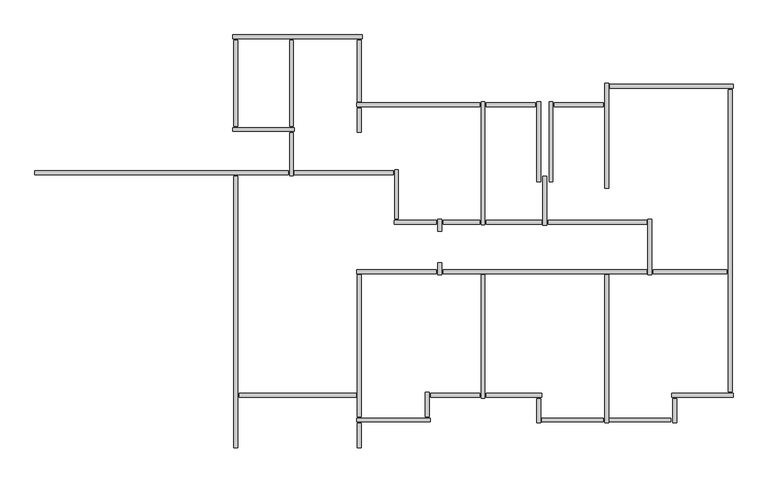
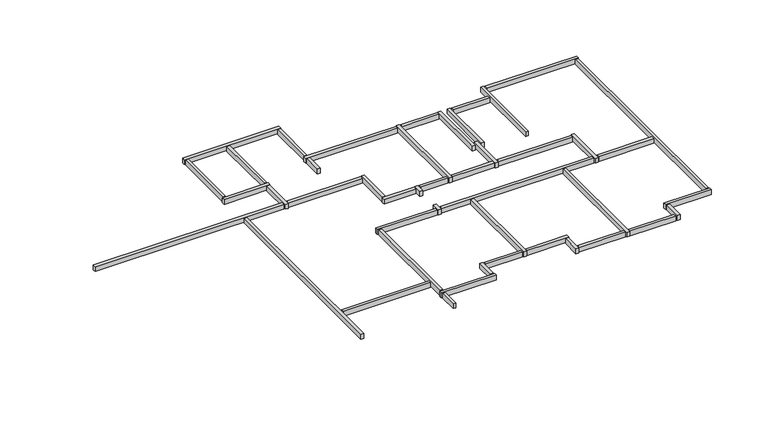
"""IFC4 building model written with IfcOpenShell, lengths in millimetres: beam geometry, Graute viga de respaldo4 : Graute viga de respaldo."""

from ifc_helpers import new_model, si_unit, frame, origin, place, context, project, spatial, polyline, outline, extrude, source, transform, mapped, element, save


def beam_ccfebb10(model_context):
    return source(origin(), model_context, "Body", "SweptSolid", [
        extrude(outline(polyline([(-54994.9587292, 57408.4278788), (-54994.9587292, 57502.4278788), (-53804.9587292, 57502.4278788), (-53804.9587292, 57408.4278788), (-54994.9587292, 57408.4278788)])), frame((0.0, 0.0, 5632.9999999), z_axis=(0.0, 0.0, 1.0), x_axis=(1.0, 0.0, 0.0)), (0.0, 0.0, 1.0), 167.0),
        extrude(outline(polyline([(-56644.9587292, 57408.4278788), (-56644.9587292, 57502.4278788), (-55454.9587292, 57502.4278788), (-55454.9587292, 57408.4278788), (-56644.9587292, 57408.4278788)])), frame((0.0, 0.0, 5632.9999999), z_axis=(0.0, 0.0, 1.0), x_axis=(1.0, 0.0, 0.0)), (0.0, 0.0, 1.0), 167.0),
        extrude(outline(polyline([(-52594.9587292, 53358.4278788), (-52594.9587292, 53452.4278788), (-50804.9587292, 53452.4278788), (-50804.9587292, 53358.4278788), (-52594.9587292, 53358.4278788)])), frame((0.0, 0.0, 5632.9999999), z_axis=(0.0, 0.0, 1.0), x_axis=(1.0, 0.0, 0.0)), (0.0, 0.0, 1.0), 167.0),
        extrude(outline(polyline([(-57994.9587292, 50358.4278788), (-57994.9587292, 50452.4278788), (-56804.9587292, 50452.4278788), (-56804.9587292, 50358.4278788), (-57994.9587292, 50358.4278788)])), frame((0.0, 0.0, 5632.9999999), z_axis=(0.0, 0.0, 1.0), x_axis=(1.0, 0.0, 0.0)), (0.0, 0.0, 1.0), 167.0),
        extrude(outline(polyline([(-58121.9587292, 50475.4278788), (-58027.9587292, 50475.4278788), (-58027.9587292, 49885.4278788), (-58121.9587292, 49885.4278788), (-58121.9587292, 50475.4278788)])), frame((0.0, 0.0, 5632.9999999), z_axis=(0.0, 0.0, 1.0), x_axis=(1.0, 0.0, 0.0)), (0.0, 0.0, 1.0), 167.0),
        extrude(outline(polyline([(-59794.9587292, 49758.4278788), (-59794.9587292, 49852.4278788), (-58004.9587292, 49852.4278788), (-58004.9587292, 49758.4278788), (-59794.9587292, 49758.4278788)])), frame((0.0, 0.0, 5632.9999999), z_axis=(0.0, 0.0, 1.0), x_axis=(1.0, 0.0, 0.0)), (0.0, 0.0, 1.0), 167.0),
        extrude(outline(polyline([(-57727.9587292, 53335.4278788), (-57821.9587292, 53335.4278788), (-57821.9587292, 53625.4278788), (-57727.9587292, 53625.4278788), (-57727.9587292, 53335.4278788)])), frame((0.0, 0.0, 5632.9999999), z_axis=(0.0, 0.0, 1.0), x_axis=(1.0, 0.0, 0.0)), (0.0, 0.0, 1.0), 167.0),
        extrude(outline(polyline([(-55144.9587292, 54558.4278788), (-55144.9587292, 54652.4278788), (-52754.9587292, 54652.4278788), (-52754.9587292, 54558.4278788), (-55144.9587292, 54558.4278788)])), frame((0.0, 0.0, 5632.9999999), z_axis=(0.0, 0.0, 1.0), x_axis=(1.0, 0.0, 0.0)), (0.0, 0.0, 1.0), 167.0),
        extrude(outline(polyline([(-56644.9587292, 54558.4278788), (-56644.9587292, 54652.4278788), (-55304.9587292, 54652.4278788), (-55304.9587292, 54558.4278788), (-56644.9587292, 54558.4278788)])), frame((0.0, 0.0, 5632.9999999), z_axis=(0.0, 0.0, 1.0), x_axis=(1.0, 0.0, 0.0)), (0.0, 0.0, 1.0), 167.0),
        extrude(outline(polyline([(-57694.9587292, 54558.4278788), (-57694.9587292, 54652.4278788), (-56804.9587292, 54652.4278788), (-56804.9587292, 54558.4278788), (-57694.9587292, 54558.4278788)])), frame((0.0, 0.0, 5632.9999999), z_axis=(0.0, 0.0, 1.0), x_axis=(1.0, 0.0, 0.0)), (0.0, 0.0, 1.0), 167.0),
        extrude(outline(polyline([(-57727.9587292, 54385.4278788), (-57821.9587292, 54385.4278788), (-57821.9587292, 54675.4278788), (-57727.9587292, 54675.4278788), (-57727.9587292, 54385.4278788)])), frame((0.0, 0.0, 5632.9999999), z_axis=(0.0, 0.0, 1.0), x_axis=(1.0, 0.0, 0.0)), (0.0, 0.0, 1.0), 167.0),
        extrude(outline(polyline([(-58884.9587292, 54558.4278788), (-58884.9587292, 54652.4278788), (-57854.9587292, 54652.4278788), (-57854.9587292, 54558.4278788), (-58884.9587292, 54558.4278788)])), frame((0.0, 0.0, 5632.9999999), z_axis=(0.0, 0.0, 1.0), x_axis=(1.0, 0.0, 0.0)), (0.0, 0.0, 1.0), 167.0),
        extrude(outline(polyline([(-58871.9587292, 55875.4278788), (-58777.9587292, 55875.4278788), (-58777.9587292, 54685.4278788), (-58871.9587292, 54685.4278788), (-58871.9587292, 55875.4278788)])), frame((0.0, 0.0, 5632.9999999), z_axis=(0.0, 0.0, 1.0), x_axis=(1.0, 0.0, 0.0)), (0.0, 0.0, 1.0), 167.0),
        extrude(outline(polyline([(-61304.9587292, 55758.4278788), (-61304.9587292, 55852.4278788), (-58904.9587292, 55852.4278788), (-58904.9587292, 55758.4278788), (-61304.9587292, 55758.4278788)])), frame((0.0, 0.0, 5632.9999999), z_axis=(0.0, 0.0, 1.0), x_axis=(1.0, 0.0, 0.0)), (0.0, 0.0, 1.0), 167.0),
        extrude(outline(polyline([(-56677.9587292, 54540.4278788), (-56771.9587292, 54540.4278788), (-56771.9587292, 57525.4278788), (-56677.9587292, 57525.4278788), (-56677.9587292, 54540.4278788)])), frame((0.0, 0.0, 5632.9999999), z_axis=(0.0, 0.0, 1.0), x_axis=(1.0, 0.0, 0.0)), (0.0, 0.0, 1.0), 167.0),
        extrude(outline(polyline([(-59794.9587292, 57408.4278788), (-59794.9587292, 57502.4278788), (-56804.9587292, 57502.4278788), (-56804.9587292, 57408.4278788), (-59794.9587292, 57408.4278788)])), frame((0.0, 0.0, 5632.9999999), z_axis=(0.0, 0.0, 1.0), x_axis=(1.0, 0.0, 0.0)), (0.0, 0.0, 1.0), 167.0),
        extrude(outline(polyline([(-59677.9587292, 56785.4278788), (-59771.9587292, 56785.4278788), (-59771.9587292, 57375.4278788), (-59677.9587292, 57375.4278788), (-59677.9587292, 56785.4278788)])), frame((0.0, 0.0, 5632.9999999), z_axis=(0.0, 0.0, 1.0), x_axis=(1.0, 0.0, 0.0)), (0.0, 0.0, 1.0), 167.0),
        extrude(outline(polyline([(-59771.9587292, 59025.4278788), (-59677.9587292, 59025.4278788), (-59677.9587292, 57535.4278788), (-59771.9587292, 57535.4278788), (-59771.9587292, 59025.4278788)])), frame((0.0, 0.0, 5632.9999999), z_axis=(0.0, 0.0, 1.0), x_axis=(1.0, 0.0, 0.0)), (0.0, 0.0, 1.0), 167.0),
        extrude(outline(polyline([(-62771.9587292, 59025.4278788), (-62677.9587292, 59025.4278788), (-62677.9587292, 56935.4278788), (-62771.9587292, 56935.4278788), (-62771.9587292, 59025.4278788)])), frame((0.0, 0.0, 5632.9999999), z_axis=(0.0, 0.0, 1.0), x_axis=(1.0, 0.0, 0.0)), (0.0, 0.0, 1.0), 167.0),
        extrude(outline(polyline([(-61421.9587292, 59025.4278788), (-61327.9587292, 59025.4278788), (-61327.9587292, 56935.4278788), (-61421.9587292, 56935.4278788), (-61421.9587292, 59025.4278788)])), frame((0.0, 0.0, 5632.9999999), z_axis=(0.0, 0.0, 1.0), x_axis=(1.0, 0.0, 0.0)), (0.0, 0.0, 1.0), 167.0),
        extrude(outline(polyline([(-61327.9587292, 55735.4278788), (-61421.9587292, 55735.4278788), (-61421.9587292, 56775.4278788), (-61327.9587292, 56775.4278788), (-61327.9587292, 55735.4278788)])), frame((0.0, 0.0, 5632.9999999), z_axis=(0.0, 0.0, 1.0), x_axis=(1.0, 0.0, 0.0)), (0.0, 0.0, 1.0), 167.0),
        extrude(outline(polyline([(-62644.9587292, 50358.4278788), (-62644.9587292, 50452.4278788), (-59804.9587292, 50452.4278788), (-59804.9587292, 50358.4278788), (-62644.9587292, 50358.4278788)])), frame((0.0, 0.0, 5632.9999999), z_axis=(0.0, 0.0, 1.0), x_axis=(1.0, 0.0, 0.0)), (0.0, 0.0, 1.0), 167.0),
        extrude(outline(polyline([(-59771.9587292, 53325.4278788), (-59677.9587292, 53325.4278788), (-59677.9587292, 49885.4278788), (-59771.9587292, 49885.4278788), (-59771.9587292, 53325.4278788)])), frame((0.0, 0.0, 5632.9999999), z_axis=(0.0, 0.0, 1.0), x_axis=(1.0, 0.0, 0.0)), (0.0, 0.0, 1.0), 167.0),
        extrude(outline(polyline([(-59794.9587292, 53358.4278788), (-59794.9587292, 53452.4278788), (-57854.9587292, 53452.4278788), (-57854.9587292, 53358.4278788), (-59794.9587292, 53358.4278788)])), frame((0.0, 0.0, 5632.9999999), z_axis=(0.0, 0.0, 1.0), x_axis=(1.0, 0.0, 0.0)), (0.0, 0.0, 1.0), 167.0),
        extrude(outline(polyline([(-57694.9587292, 53358.4278788), (-57694.9587292, 53452.4278788), (-52754.9587292, 53452.4278788), (-52754.9587292, 53358.4278788), (-57694.9587292, 53358.4278788)])), frame((0.0, 0.0, 5632.9999999), z_axis=(0.0, 0.0, 1.0), x_axis=(1.0, 0.0, 0.0)), (0.0, 0.0, 1.0), 167.0),
        extrude(outline(polyline([(-56677.9587292, 50335.4278788), (-56771.9587292, 50335.4278788), (-56771.9587292, 53325.4278788), (-56677.9587292, 53325.4278788), (-56677.9587292, 50335.4278788)])), frame((0.0, 0.0, 5632.9999999), z_axis=(0.0, 0.0, 1.0), x_axis=(1.0, 0.0, 0.0)), (0.0, 0.0, 1.0), 167.0),
        extrude(outline(polyline([(-55304.9587292, 50452.4278788), (-55304.9587292, 50358.4278788), (-56644.9587292, 50358.4278788), (-56644.9587292, 50452.4278788), (-55304.9587292, 50452.4278788)])), frame((0.0, 0.0, 5632.9999999), z_axis=(0.0, 0.0, 1.0), x_axis=(1.0, 0.0, 0.0)), (0.0, 0.0, 1.0), 167.0),
        extrude(outline(polyline([(-55327.9587292, 49735.4278788), (-55421.9587292, 49735.4278788), (-55421.9587292, 50325.4278788), (-55327.9587292, 50325.4278788), (-55327.9587292, 49735.4278788)])), frame((0.0, 0.0, 5632.9999999), z_axis=(0.0, 0.0, 1.0), x_axis=(1.0, 0.0, 0.0)), (0.0, 0.0, 1.0), 167.0),
        extrude(outline(polyline([(-55294.9587292, 49758.4278788), (-55294.9587292, 49852.4278788), (-53804.9587292, 49852.4278788), (-53804.9587292, 49758.4278788), (-55294.9587292, 49758.4278788)])), frame((0.0, 0.0, 5632.9999999), z_axis=(0.0, 0.0, 1.0), x_axis=(1.0, 0.0, 0.0)), (0.0, 0.0, 1.0), 167.0),
        extrude(outline(polyline([(-52165.9809043, 49853.4278788), (-52165.9809043, 49758.4278788), (-53654.9587292, 49758.4278788), (-53654.9587292, 49853.4278788), (-52165.9809043, 49853.4278788)])), frame((0.0, 0.0, 5617.1856208), z_axis=(0.0, 0.0, 1.0), x_axis=(1.0, 0.0, 0.0)), (0.0, 0.0, 1.0), 165.0),
        extrude(outline(polyline([(-50771.9587292, 57825.4278788), (-50677.9587292, 57825.4278788), (-50677.9587292, 50485.4278788), (-50771.9587292, 50485.4278788), (-50771.9587292, 57825.4278788)])), frame((0.0, 0.0, 5632.9999999), z_axis=(0.0, 0.0, 1.0), x_axis=(1.0, 0.0, 0.0)), (0.0, 0.0, 1.0), 167.0),
        extrude(outline(polyline([(-52721.9587292, 54675.4278788), (-52627.9587292, 54675.4278788), (-52627.9587292, 53330.0746661), (-52721.9587292, 53330.0746661), (-52721.9587292, 54675.4278788)])), frame((0.0, 0.0, 5632.9999999), z_axis=(0.0, 0.0, 1.0), x_axis=(1.0, 0.0, 0.0)), (0.0, 0.0, 1.0), 167.0),
        extrude(outline(polyline([(-55271.9587292, 55725.4278788), (-55177.9587292, 55725.4278788), (-55177.9587292, 54535.4278788), (-55271.9587292, 54535.4278788), (-55271.9587292, 55725.4278788)])), frame((0.0, 0.0, 5632.9999999), z_axis=(0.0, 0.0, 1.0), x_axis=(1.0, 0.0, 0.0)), (0.0, 0.0, 1.0), 167.0),
        extrude(outline(polyline([(-55121.9587292, 57525.4278788), (-55027.9587292, 57525.4278788), (-55027.9587292, 55585.4278788), (-55121.9587292, 55585.4278788), (-55121.9587292, 57525.4278788)])), frame((0.0, 0.0, 5632.9999999), z_axis=(0.0, 0.0, 1.0), x_axis=(1.0, 0.0, 0.0)), (0.0, 0.0, 1.0), 167.0),
        extrude(outline(polyline([(-55421.9587292, 57525.4278788), (-55327.9587292, 57525.4278788), (-55327.9587292, 55585.4278788), (-55421.9587292, 55585.4278788), (-55421.9587292, 57525.4278788)])), frame((0.0, 0.0, 5632.9999999), z_axis=(0.0, 0.0, 1.0), x_axis=(1.0, 0.0, 0.0)), (0.0, 0.0, 1.0), 167.0),
        extrude(outline(polyline([(-53771.9587292, 57975.4278788), (-53677.9587292, 57975.4278788), (-53677.9587292, 55435.4278788), (-53771.9587292, 55435.4278788), (-53771.9587292, 57975.4278788)])), frame((0.0, 0.0, 5632.9999999), z_axis=(0.0, 0.0, 1.0), x_axis=(1.0, 0.0, 0.0)), (0.0, 0.0, 1.0), 167.0),
        extrude(outline(polyline([(-50654.9587292, 57952.4278788), (-50654.9587292, 57858.4278788), (-53644.9587292, 57858.4278788), (-53644.9587292, 57952.4278788), (-50654.9587292, 57952.4278788)])), frame((0.0, 0.0, 5632.9999999), z_axis=(0.0, 0.0, 1.0), x_axis=(1.0, 0.0, 0.0)), (0.0, 0.0, 1.0), 167.0),
        extrude(outline(polyline([(-52027.9587292, 49735.4278788), (-52121.9587292, 49735.4278788), (-52121.9587292, 50325.4278788), (-52027.9587292, 50325.4278788), (-52027.9587292, 49735.4278788)])), frame((0.0, 0.0, 5632.9999999), z_axis=(0.0, 0.0, 1.0), x_axis=(1.0, 0.0, 0.0)), (0.0, 0.0, 1.0), 167.0),
        extrude(outline(polyline([(-52144.9587292, 50358.4278788), (-52144.9587292, 50452.4278788), (-50654.9587292, 50452.4278788), (-50654.9587292, 50358.4278788), (-52144.9587292, 50358.4278788)])), frame((0.0, 0.0, 5632.9999999), z_axis=(0.0, 0.0, 1.0), x_axis=(1.0, 0.0, 0.0)), (0.0, 0.0, 1.0), 167.0),
        extrude(outline(polyline([(-53677.9587292, 49735.4278788), (-53771.9587292, 49735.4278788), (-53771.9587292, 53325.4278788), (-53677.9587292, 53325.4278788), (-53677.9587292, 49735.4278788)])), frame((0.0, 0.0, 5632.9999999), z_axis=(0.0, 0.0, 1.0), x_axis=(1.0, 0.0, 0.0)), (0.0, 0.0, 1.0), 167.0),
        extrude(outline(polyline([(-59677.9587292, 49135.4278788), (-59771.9587292, 49135.4278788), (-59771.9587292, 49725.4278788), (-59677.9587292, 49725.4278788), (-59677.9587292, 49135.4278788)])), frame((0.0, 0.0, 5632.9999999), z_axis=(0.0, 0.0, 1.0), x_axis=(1.0, 0.0, 0.0)), (0.0, 0.0, 1.0), 167.0),
        extrude(outline(polyline([(-62794.9587292, 56808.4278788), (-62794.9587292, 56902.4278788), (-61304.9587292, 56902.4278788), (-61304.9587292, 56808.4278788), (-62794.9587292, 56808.4278788)])), frame((0.0, 0.0, 5632.9999999), z_axis=(0.0, 0.0, 1.0), x_axis=(1.0, 0.0, 0.0)), (0.0, 0.0, 1.0), 167.0),
        extrude(outline(polyline([(-62794.9587292, 59058.4278788), (-62794.9587292, 59152.4278788), (-59654.9587292, 59152.4278788), (-59654.9587292, 59058.4278788), (-62794.9587292, 59058.4278788)])), frame((0.0, 0.0, 5632.9999999), z_axis=(0.0, 0.0, 1.0), x_axis=(1.0, 0.0, 0.0)), (0.0, 0.0, 1.0), 167.0),
        extrude(outline(polyline([(-67601.7587292, 55758.4278788), (-67601.7587292, 55852.4278788), (-61454.9587292, 55852.4278788), (-61454.9587292, 55758.4278788), (-67601.7587292, 55758.4278788)])), frame((0.0, 0.0, 5632.9999999), z_axis=(0.0, 0.0, 1.0), x_axis=(1.0, 0.0, 0.0)), (0.0, 0.0, 1.0), 167.0),
        extrude(outline(polyline([(-62677.9587292, 49132.8979841), (-62771.9587292, 49132.8979841), (-62771.9587292, 55725.4278788), (-62677.9587292, 55725.4278788), (-62677.9587292, 49132.8979841)])), frame((0.0, 0.0, 5632.9999999), z_axis=(0.0, 0.0, 1.0), x_axis=(1.0, 0.0, 0.0)), (0.0, 0.0, 1.0), 167.0),
    ])


if __name__ == "__main__":
    model = new_model("IFC4")
    model_context = context("Model", 3, world=origin())
    ifc_project = project(units=[si_unit("LENGTHUNIT", "METRE", prefix="MILLI")], contexts=[model_context])
    site = spatial("IfcSite", under=ifc_project)
    building = spatial("IfcBuilding", under=site)
    placement = place(None, origin())
    beam_shape = beam_ccfebb10(model_context)
    element("IfcBeam", 1, ObjectType="Graute viga de respaldo4 : Graute viga de respaldo", at=placement, inside=building, context=model_context, shape_type="MappedRepresentation", body=[
        mapped(beam_shape, transform((0.0, 0.0, 0.0), x_axis=(1.0, 0.0, 0.0), y_axis=(0.0, 1.0, 0.0), z_axis=(0.0, 0.0, 1.0))),
    ])
    save(model, "model.ifc")

# Revit data of these elements
# Element 1 (IfcBeam, "Graute viga de respaldo4 : Graute viga de respaldo")
#   Materials on its faces: "Concreto, Faixa de areia/cimento"
# Materials
#   "Concreto, Faixa de areia/cimento": class "Concreto", colour RGB 127 127 127, transparency 0, Description = "Revestimento de laje de concreto", Cost = 0
